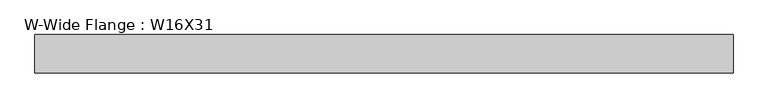
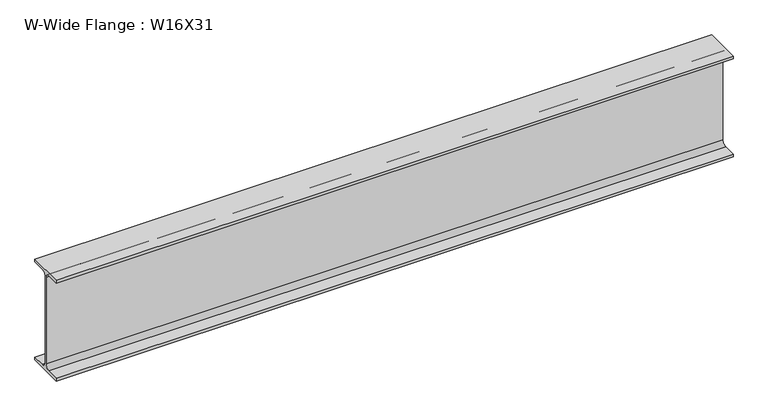
"""IFC4 building model written with IfcOpenShell, lengths in millimetres: beam geometry, W-Wide Flange : W16X31."""

from ifc_helpers import new_model, si_unit, point, frame, frame_2d, origin, place, context, project, spatial, polyline, circle_curve, trimmed, segment, composite_curve, outline, extrude, source, transform, mapped, element, save


def w_wide_flange_w16x31_3178c40c(model_context):
    return source(origin(), model_context, "Body", "SweptSolid", [
        extrude(outline(composite_curve([segment(polyline([(70.231, -190.754), (70.231, -201.93), (-70.231, -201.93), (-70.231, -190.754), (-20.8915, -190.754)]), True, "CONTINUOUS"), segment(trimmed(circle_curve(frame_2d((-20.8915, -173.355)), 17.399), [point((-20.8915, -190.754))], [point((-3.4925, -173.355))], True, "CARTESIAN"), True, "CONTINUOUS"), segment(polyline([(-3.4925, -173.355), (-3.4925, 173.355)]), True, "CONTINUOUS"), segment(trimmed(circle_curve(frame_2d((-20.8915, 173.355)), 17.399), [point((-3.4925, 173.355))], [point((-20.8915, 190.754))], True, "CARTESIAN"), True, "CONTINUOUS"), segment(polyline([(-20.8915, 190.754), (-70.231, 190.754), (-70.231, 201.93), (70.231, 201.93), (70.231, 190.754), (20.8915, 190.754)]), True, "CONTINUOUS"), segment(trimmed(circle_curve(frame_2d((20.8915, 173.355)), 17.399), [point((20.8915, 190.754))], [point((3.4925, 173.355))], True, "CARTESIAN"), True, "CONTINUOUS"), segment(polyline([(3.4925, 173.355), (3.4925, -173.355)]), True, "CONTINUOUS"), segment(trimmed(circle_curve(frame_2d((20.8915, -173.355)), 17.399), [point((3.4925, -173.355))], [point((20.8915, -190.754))], True, "CARTESIAN"), True, "CONTINUOUS"), segment(polyline([(20.8915, -190.754), (70.231, -190.754)]), True, "CONTINUOUS")], self_intersect=False)), frame((-1282.7, 0.0, 0.0), z_axis=(1.0, 0.0, 0.0), x_axis=(0.0, 1.0, 0.0)), (0.0, 0.0, 1.0), 2565.4),
    ])


if __name__ == "__main__":
    model = new_model("IFC4")
    model_context = context("Model", 3, world=origin())
    ifc_project = project(units=[si_unit("LENGTHUNIT", "METRE", prefix="MILLI")], contexts=[model_context])
    site = spatial("IfcSite", under=ifc_project)
    building = spatial("IfcBuilding", under=site)
    placement = place(None, origin())
    w_wide_flange_w16x31_shape = w_wide_flange_w16x31_3178c40c(model_context)
    element("IfcBeam", 1, ObjectType="W-Wide Flange : W16X31", at=placement, inside=building, context=model_context, shape_type="MappedRepresentation", body=[
        mapped(w_wide_flange_w16x31_shape, transform((0.0, 0.0, 0.0), x_axis=(1.0, 0.0, 0.0), y_axis=(0.0, 1.0, 0.0), z_axis=(0.0, 0.0, 1.0))),
    ])
    save(model, "model.ifc")

# Revit data of these elements
# Type "W-Wide Flange : W16X31"
#   Assembly Code = "B10"
#   W = 31
#   Length [instance default] = 5' - 0"
#   bf = 0' - 5.53"
#   d = 1' - 3.9"
#   k = 0' - 1 1/8"
#   k2 = 0' - 0.685"
#   tf = 0' - 0.44"
#   tw = 0' - 0.275"
#   A = 0.0634028 SF
#   Structural Material [instance default] = Steel ASTM A992
# Element 1 (IfcBeam, "W-Wide Flange : W16X31")
#   Materials on its faces: "Steel ASTM A992"
# Materials
#   "Steel ASTM A992": class "Metal", colour RGB 199 199 199, transparency 0, Description = "Structural steel 50ksi", Cost = 0
